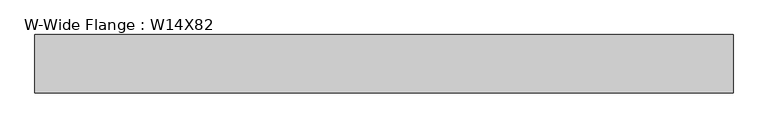
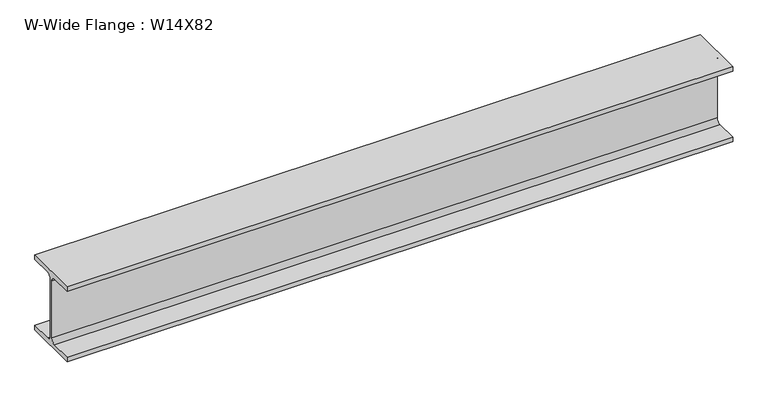
"""IFC4 building model written with IfcOpenShell, lengths in millimetres: beam geometry, W-Wide Flange : W14X82."""

from ifc_helpers import new_model, si_unit, point, frame, frame_2d, origin, place, context, project, spatial, polyline, circle_curve, trimmed, segment, composite_curve, outline, extrude, source, transform, mapped, element, save


def w_wide_flange_w14x82_8d14bb68(model_context):
    return source(origin(), model_context, "Body", "SweptSolid", [
        extrude(outline(composite_curve([segment(polyline([(128.27, -159.893), (128.27, -181.61), (-128.27, -181.61), (-128.27, -159.893), (-27.6225, -159.893)]), True, "CONTINUOUS"), segment(trimmed(circle_curve(frame_2d((-27.6225, -138.7475)), 21.1455), [point((-27.6225, -159.893))], [point((-6.477, -138.7475))], True, "CARTESIAN"), True, "CONTINUOUS"), segment(polyline([(-6.477, -138.7475), (-6.477, 138.7475)]), True, "CONTINUOUS"), segment(trimmed(circle_curve(frame_2d((-27.6225, 138.7475)), 21.1455), [point((-6.477, 138.7475))], [point((-27.6225, 159.893))], True, "CARTESIAN"), True, "CONTINUOUS"), segment(polyline([(-27.6225, 159.893), (-128.27, 159.893), (-128.27, 181.61), (128.27, 181.61), (128.27, 159.893), (27.6225, 159.893)]), True, "CONTINUOUS"), segment(trimmed(circle_curve(frame_2d((27.6225, 138.7475)), 21.1455), [point((27.6225, 159.893))], [point((6.477, 138.7475))], True, "CARTESIAN"), True, "CONTINUOUS"), segment(polyline([(6.477, 138.7475), (6.477, -138.7475)]), True, "CONTINUOUS"), segment(trimmed(circle_curve(frame_2d((27.6225, -138.7475)), 21.1455), [point((6.477, -138.7475))], [point((27.6225, -159.893))], True, "CARTESIAN"), True, "CONTINUOUS"), segment(polyline([(27.6225, -159.893), (128.27, -159.893)]), True, "CONTINUOUS")], self_intersect=False)), frame((-1530.35, 0.0, 0.0), z_axis=(1.0, 0.0, 0.0), x_axis=(0.0, 1.0, 0.0)), (0.0, 0.0, 1.0), 3060.7),
    ])


if __name__ == "__main__":
    model = new_model("IFC4")
    model_context = context("Model", 3, world=origin())
    ifc_project = project(units=[si_unit("LENGTHUNIT", "METRE", prefix="MILLI")], contexts=[model_context])
    site = spatial("IfcSite", under=ifc_project)
    building = spatial("IfcBuilding", under=site)
    placement = place(None, origin())
    w_wide_flange_w14x82_shape = w_wide_flange_w14x82_8d14bb68(model_context)
    element("IfcBeam", 1, ObjectType="W-Wide Flange : W14X82", at=placement, inside=building, context=model_context, shape_type="MappedRepresentation", body=[
        mapped(w_wide_flange_w14x82_shape, transform((0.0, 0.0, 0.0), x_axis=(1.0, 0.0, 0.0), y_axis=(0.0, 1.0, 0.0), z_axis=(0.0, 0.0, 1.0))),
    ])
    save(model, "model.ifc")

# Revit data of these elements
# Type "W-Wide Flange : W14X82"
#   Assembly Code = "B10"
#   W = 82
#   Length [instance default] = 5' - 0"
#   bf = 0' - 10.1"
#   d = 1' - 2.3"
#   k = 0' - 1 11/16"
#   k2 = 0' - 0.8325"
#   tf = 0' - 0.855"
#   tw = 0' - 0.51"
#   A = 0.166667 SF
#   Structural Material [instance default] = _STRUCTURAL STEEL (SEE STRUCT. DWGS)
# Element 1 (IfcBeam, "W-Wide Flange : W14X82")
#   Materials on its faces: "_STRUCTURAL STEEL (SEE STRUCT. DWGS)"
# Materials
#   "_STRUCTURAL STEEL (SEE STRUCT. DWGS)": class "Metal", colour RGB 199 199 199, transparency 0, Description = "Structural steel 50ksi", Cost = 0
